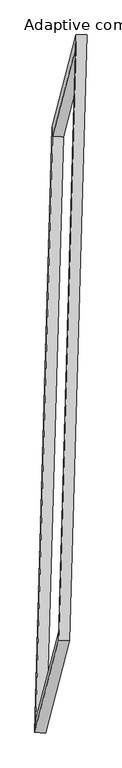
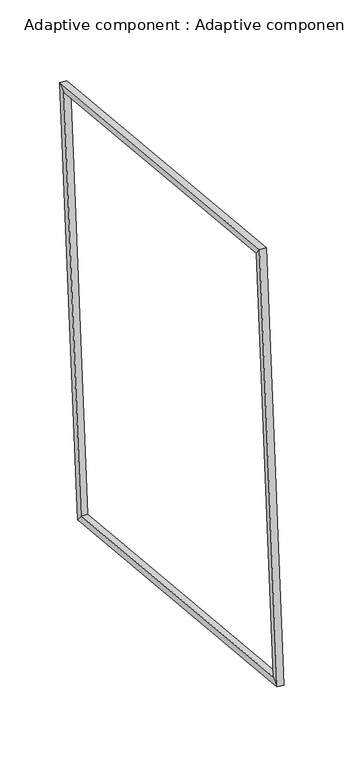
"""IFC4 building model written with IfcOpenShell, lengths in millimetres: proxy geometry, Adaptive component : Adaptive component."""

import ifcopenshell
import ifcopenshell.guid

model = None  # the IFC model being written
_history = None  # IfcOwnerHistory: only IFC2X3 demands one
_inside = {}  # id of a spatial element -> (the spatial element, [elements in it])
_under = {}  # id of a project, library or spatial element -> (it, [spatial elements below it])
_declared = {}  # id of a project -> (the project, [libraries it declares])
_typed = {}  # id of a type object -> (the type object, [elements of that type])
_made_of = {}  # id of a material, layer set ... -> (it, [elements and type objects made of it])


def new_model(schema):
    """Start an empty IFC model of exactly this schema.

    Asked for "IFC4X3", IfcOpenShell would pick the latest addendum, in which some entities
    have other attributes; the version numbers below select the first issue.
    IFC2X3 requires an IfcOwnerHistory on every rooted entity: one is made here for all.
    """
    global model, _history
    if schema == "IFC4X3":
        model = ifcopenshell.file(schema_version=(4, 3, 0, 0))
    else:
        model = ifcopenshell.file(schema=schema)
    _inside.clear()
    _under.clear()
    _declared.clear()
    _typed.clear()
    _made_of.clear()
    _history = None
    if model.schema == "IFC2X3":
        org = make("IfcOrganization", Name="unknown")
        user = make(
            "IfcPersonAndOrganization",
            ThePerson=make("IfcPerson", FamilyName="unknown"),
            TheOrganization=org,
        )
        app = make(
            "IfcApplication",
            ApplicationDeveloper=org,
            Version="unknown",
            ApplicationFullName="unknown",
            ApplicationIdentifier="unknown",
        )
        _history = make(
            "IfcOwnerHistory",
            OwningUser=user,
            OwningApplication=app,
            ChangeAction="ADDED",
            CreationDate=0,
        )
    return model


def make(cls, **values):
    """One entity of the class cls with the attributes given. An attribute that is None is left unset."""
    return model.create_entity(
        cls, **{name: value for name, value in values.items() if value is not None}
    )


def rooted(cls, **values):
    """An entity with a GlobalId (a new one), such as an element, a storey or a relation."""
    return make(cls, GlobalId=ifcopenshell.guid.new(), OwnerHistory=_history, **values)


def si_unit(unit_type, name, prefix=None):
    """IfcSIUnit, for example si_unit("LENGTHUNIT", "METRE", prefix="MILLI")."""
    return make("IfcSIUnit", UnitType=unit_type, Prefix=prefix, Name=name)


def assignment(units):
    """IfcUnitAssignment: the units of a project."""
    return None if units is None else make("IfcUnitAssignment", Units=units)


def point(xyz):
    """IfcCartesianPoint."""
    return None if xyz is None else make("IfcCartesianPoint", Coordinates=xyz)


def direction(xyz):
    """IfcDirection."""
    return None if xyz is None else make("IfcDirection", DirectionRatios=xyz)


def frame(location, z_axis=None, x_axis=None):
    """IfcAxis2Placement3D, a coordinate frame: its origin and axes. An axis left out is left unset."""
    return make(
        "IfcAxis2Placement3D",
        Location=point(location),
        Axis=direction(z_axis),
        RefDirection=direction(x_axis),
    )


def origin():
    """The frame at (0, 0, 0) with its axes left unset."""
    return frame((0.0, 0.0, 0.0))


def place(relative_to, where):
    """IfcLocalPlacement: puts the frame where relative to a parent placement (None: the world)."""
    return make(
        "IfcLocalPlacement", PlacementRelTo=relative_to, RelativePlacement=where
    )


def context(
    kind, dimensions, precision=None, world=None, true_north=None, identifier=None
):
    """IfcGeometricRepresentationContext, for example the 3D "Model" context."""
    return make(
        "IfcGeometricRepresentationContext",
        ContextIdentifier=identifier,
        ContextType=kind,
        CoordinateSpaceDimension=dimensions,
        Precision=precision,
        WorldCoordinateSystem=world,
        TrueNorth=true_north,
    )


def project(units=None, contexts=None):
    """IfcProject with its units and contexts."""
    return rooted(
        "IfcProject",
        Name="project",
        RepresentationContexts=contexts,
        UnitsInContext=assignment(units),
    )


def spatial(cls, under=None, at=None, **own):
    """A site, building, storey or space (cls), placed at a placement, below another one or the project."""
    s = rooted(cls, ObjectPlacement=at, **own)
    if under is not None:
        _under.setdefault(under.id(), (under, []))[1].append(s)
    return s


def faces_of(points, faces, orient=None, outer=None):
    """IfcFace entities. A face is a list of loops; a loop is a list of indices into points, from 0.

    orient and outer hold one flag for each loop. By default every Orientation is true, the
    first loop of a face is its IfcFaceOuterBound and the others are IfcFaceBound.
    """
    made = []
    for i, loops in enumerate(faces):
        bounds = []
        for j, loop in enumerate(loops):
            is_outer = j == 0 if outer is None else outer[i][j]
            bounds.append(
                make(
                    "IfcFaceOuterBound" if is_outer else "IfcFaceBound",
                    Bound=make("IfcPolyLoop", Polygon=[points[k] for k in loop]),
                    Orientation=True if orient is None else orient[i][j],
                )
            )
        made.append(make("IfcFace", Bounds=bounds))
    return made


def faceted_brep(points, faces, orient=None, outer=None, voids=None):
    """IfcFacetedBrep: a solid bounded by flat faces; with voids (closed shells), ...WithVoids."""
    shared = [point(p) for p in points]
    hull = make("IfcClosedShell", CfsFaces=faces_of(shared, faces, orient, outer))
    if voids is None:
        return make("IfcFacetedBrep", Outer=hull)
    return make(
        "IfcFacetedBrepWithVoids",
        Outer=hull,
        Voids=[
            make(cls, CfsFaces=faces_of(shared, fs, o, b)) for cls, fs, o, b in voids
        ],
    )


def shape(context_of_items, identifier, shape_type, items):
    """IfcShapeRepresentation: the items that make up one representation, for example the "Body"."""
    return make(
        "IfcShapeRepresentation",
        ContextOfItems=context_of_items,
        RepresentationIdentifier=identifier,
        RepresentationType=shape_type,
        Items=items,
    )


def source(mapping_origin, context_of_items, identifier, shape_type, items):
    """IfcRepresentationMap: a shape defined once, which mapped items show again and again."""
    return make(
        "IfcRepresentationMap",
        MappingOrigin=mapping_origin,
        MappedRepresentation=shape(context_of_items, identifier, shape_type, items),
    )


def transform(
    local_origin,
    x_axis=None,
    y_axis=None,
    z_axis=None,
    scale=None,
    scale2=None,
    scale3=None,
    uniform=True,
):
    """IfcCartesianTransformationOperator3D, or its non-uniform kind. x_axis, y_axis, z_axis: its Axis1, 2, 3."""
    if uniform:
        return make(
            "IfcCartesianTransformationOperator3D",
            Axis1=direction(x_axis),
            Axis2=direction(y_axis),
            LocalOrigin=point(local_origin),
            Scale=scale,
            Axis3=direction(z_axis),
        )
    return make(
        "IfcCartesianTransformationOperator3DnonUniform",
        Axis1=direction(x_axis),
        Axis2=direction(y_axis),
        LocalOrigin=point(local_origin),
        Scale=scale,
        Axis3=direction(z_axis),
        Scale2=scale2,
        Scale3=scale3,
    )


def mapped(mapping_source, mapping_target):
    """IfcMappedItem: shows the shape of a source again, moved by a transform."""
    return make(
        "IfcMappedItem", MappingSource=mapping_source, MappingTarget=mapping_target
    )


def made_of(thing, what):
    """Note that an element or type object is made of a material, layer set ...; save() writes the relation."""
    if what is not None:
        _made_of.setdefault(what.id(), (what, []))[1].append(thing)
    return thing


def element(
    cls,
    number,
    at=None,
    inside=None,
    cuts=None,
    type_object=None,
    material=None,
    context=None,
    identifier="Body",
    shape_type=None,
    held_by="IfcProductDefinitionShape",
    body=None,
    shapes=None,
    **own,
):
    """One element of the class cls, such as IfcWall. Its Tag is "e" and its number.

    at: its placement. inside: the storey or other place that contains it. cuts: it is an
    opening in that element (IfcRelVoidsElement). A single representation is given by context,
    identifier, shape_type and body (its items); several are given by shapes. held_by: the class
    of the entity that holds the representations. save() writes the other relations.
    """
    e = rooted(cls, Tag="e%d" % number, ObjectPlacement=at, **own)
    if body is not None:
        shapes = [shape(context, identifier, shape_type, body)]
    if shapes is not None:
        e.Representation = make(held_by, Representations=shapes)
    if inside is not None:
        _inside.setdefault(inside.id(), (inside, []))[1].append(e)
    if cuts is not None:
        rooted(
            "IfcRelVoidsElement", RelatingBuildingElement=cuts, RelatedOpeningElement=e
        )
    if type_object is not None:
        _typed.setdefault(type_object.id(), (type_object, []))[1].append(e)
    return made_of(e, material)


def aggregate(whole, parts):
    """IfcRelAggregates: a whole, such as a stair, and the parts it consists of."""
    return rooted("IfcRelAggregates", RelatingObject=whole, RelatedObjects=parts)


def save(model, path):
    """Write the relations noted so far, then the file.

    IfcRelAggregates (storeys below a building ...), IfcRelContainedInSpatialStructure (elements
    in a storey), IfcRelDefinesByType, IfcRelAssociatesMaterial and IfcRelDeclares: one each for
    every whole, place, type object, material and project.
    """
    for whole, parts in _under.values():
        aggregate(whole, parts)
    for where, things in _inside.values():
        rooted(
            "IfcRelContainedInSpatialStructure",
            RelatedElements=things,
            RelatingStructure=where,
        )
    for kind, things in _typed.values():
        rooted("IfcRelDefinesByType", RelatedObjects=things, RelatingType=kind)
    for what, things in _made_of.values():
        rooted("IfcRelAssociatesMaterial", RelatedObjects=things, RelatingMaterial=what)
    for by, libraries in _declared.values():
        rooted("IfcRelDeclares", RelatingContext=by, RelatedDefinitions=libraries)
    model.write(path)


def adaptive_component_adaptive_component_60bdf796(model_context):
    return source(origin(), model_context, "Body", "Brep", [
        faceted_brep([(101.4783472, 1653.2432234, 3197.4782263), (166.5017696, 1653.1219261, 3197.0805704), (23.4933562, 1104.6786645, -984.195658), (-41.4084636, 1105.2663129, -980.2425882), (99.2076857, 1580.3502622, 3141.5475372), (-39.2748254, 1049.2640258, -907.4004773), (164.2311081, 1580.2289649, 3141.1498812), (25.6269945, 1048.6763774, -911.3535471), (-80.5544695, -2495.8347466, -508.3703539), (-145.3535411, -2491.6915544, -504.8871664), (-139.4984837, -2418.9163356, -449.0636273), (-74.6994122, -2423.0595278, -452.5468147), (62.4539439, -1947.391485, 3672.9058745), (-2.4667303, -1943.7146439, 3672.8336481), (-1.0159726, -1887.8300993, 3599.8843872), (63.9047015, -1891.5069404, 3599.9566136)], [[[0, 1, 2, 3]], [[4, 0, 3, 5]], [[6, 4, 5, 7]], [[1, 6, 7, 2]], [[3, 2, 8, 9]], [[5, 3, 9, 10]], [[7, 5, 10, 11]], [[2, 7, 11, 8]], [[9, 8, 12, 13]], [[10, 9, 13, 14]], [[11, 10, 14, 15]], [[8, 11, 15, 12]], [[13, 12, 1, 0]], [[14, 13, 0, 4]], [[15, 14, 4, 6]], [[12, 15, 6, 1]]]),
    ])


if __name__ == "__main__":
    model = new_model("IFC4")
    model_context = context("Model", 3, world=origin())
    ifc_project = project(units=[si_unit("LENGTHUNIT", "METRE", prefix="MILLI")], contexts=[model_context])
    site = spatial("IfcSite", under=ifc_project)
    building = spatial("IfcBuilding", under=site)
    placement = place(None, origin())
    adaptive_component_adaptive_component_shape = adaptive_component_adaptive_component_60bdf796(model_context)
    element("IfcBuildingElementProxy", 1, Name="Adaptive component : Adaptive component", ObjectType="Adaptive component : Adaptive component", at=placement, inside=building, context=model_context, shape_type="MappedRepresentation", body=[
        mapped(adaptive_component_adaptive_component_shape, transform((0.0, 0.0, 0.0), x_axis=(1.0, 0.0, 0.0), y_axis=(0.0, 1.0, 0.0), z_axis=(0.0, 0.0, 1.0))),
    ])
    save(model, "model.ifc")

# Revit data of these elements
# Type "Adaptive component : Adaptive component"
#   r [instance default] = 2063.125 mm
#   2r [instance default] = 4126.251 mm
#   Number [instance default] = 5
#   Default Elevation = 0
# Element 1 (IfcBuildingElementProxy, "Adaptive component : Adaptive component")
#   r = 2690.125 mm
#   2r = 5380.25 mm
#   Number = 27
